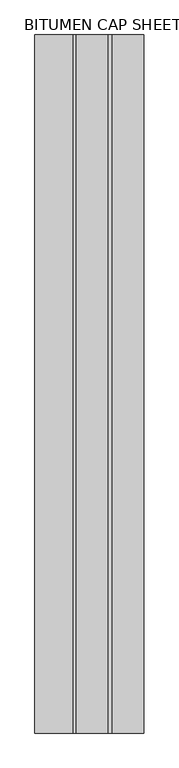
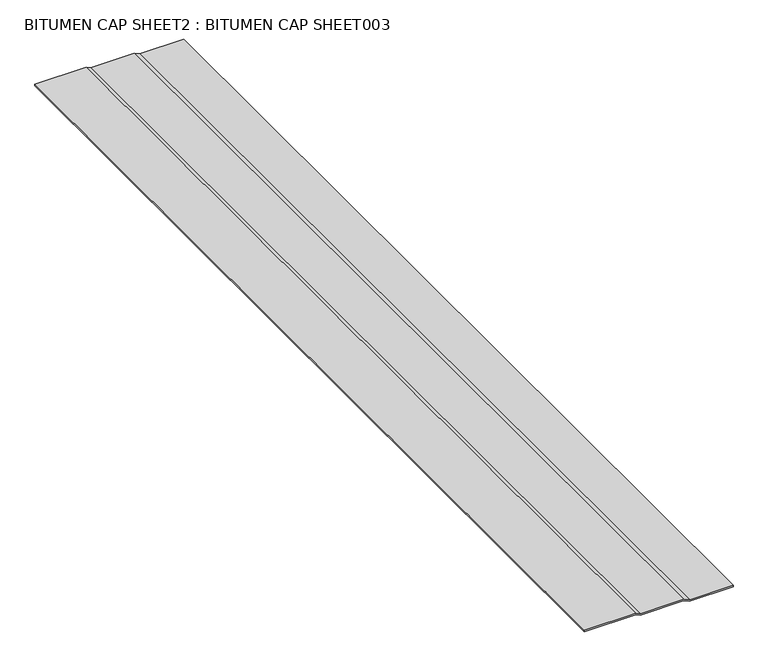
"""IFC4 building model written with IfcOpenShell, lengths in millimetres: proxy geometry, BITUMEN CAP SHEET2 : BITUMEN CAP SHEET003."""

from ifc_helpers import new_model, si_unit, frame, origin, place, context, project, spatial, polyline, outline, extrude, source, transform, mapped, element, save


def bitumen_cap_sheet2_bitumen_cap_sheet003_03d49bda(model_context):
    return source(origin(), model_context, "Body", "SweptSolid", [
        extrude(outline(polyline([(40259.2002678, -2469.2761954), (40262.3752678, -2469.2761954), (40262.3752678, -2560.795457), (40267.6612773, -2573.2602756), (40267.6612773, -2663.9440313), (40271.9940719, -2673.6609328), (40271.9940719, -2781.5474293), (40268.8188423, -2781.5474293), (40268.8188423, -2674.3362183), (40264.4862773, -2664.6198318), (40264.4862773, -2573.9056756), (40259.2002678, -2561.440857), (40259.2002678, -2469.2761954)])), frame((0.0, 999.75, 0.0), z_axis=(0.0, 1.0, 0.0), x_axis=(0.0, 0.0, 1.0)), (0.0, 0.0, 1.0), 2000.25),
    ])


if __name__ == "__main__":
    model = new_model("IFC4")
    model_context = context("Model", 3, world=origin())
    ifc_project = project(units=[si_unit("LENGTHUNIT", "METRE", prefix="MILLI")], contexts=[model_context])
    site = spatial("IfcSite", under=ifc_project)
    building = spatial("IfcBuilding", under=site)
    placement = place(None, origin())
    bitumen_cap_sheet2_bitumen_cap_sheet003_shape = bitumen_cap_sheet2_bitumen_cap_sheet003_03d49bda(model_context)
    element("IfcBuildingElementProxy", 1, Name="BITUMEN CAP SHEET2 : BITUMEN CAP SHEET003", ObjectType="BITUMEN CAP SHEET2 : BITUMEN CAP SHEET003", at=placement, inside=building, context=model_context, shape_type="MappedRepresentation", body=[
        mapped(bitumen_cap_sheet2_bitumen_cap_sheet003_shape, transform((0.0, 0.0, 0.0), x_axis=(1.0, 0.0, 0.0), y_axis=(0.0, 1.0, 0.0), z_axis=(0.0, 0.0, 1.0))),
    ])
    save(model, "model.ifc")

# Revit data of these elements
# Type "BITUMEN CAP SHEET2 : BITUMEN CAP SHEET003"
#   NameOverride = "BITUMEN CAP SHEET003"
# Element 1 (IfcBuildingElementProxy, "BITUMEN CAP SHEET2 : BITUMEN CAP SHEET003")
#   Materials on its faces: "MODIFIED BITUMEN GRANULE SURFACED CAP SHEET"
# Materials
#   "MODIFIED BITUMEN GRANULE SURFACED CAP SHEET": class "Unassigned", colour RGB 85 85 127, transparency 0
